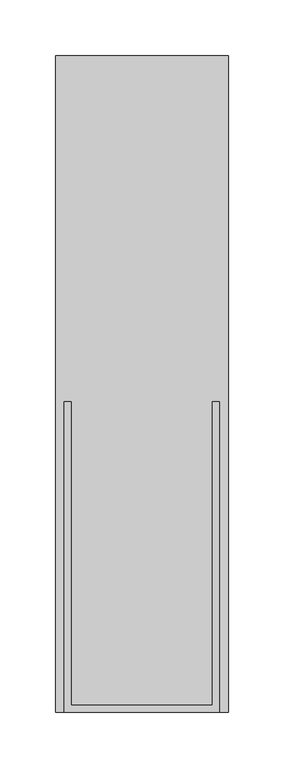
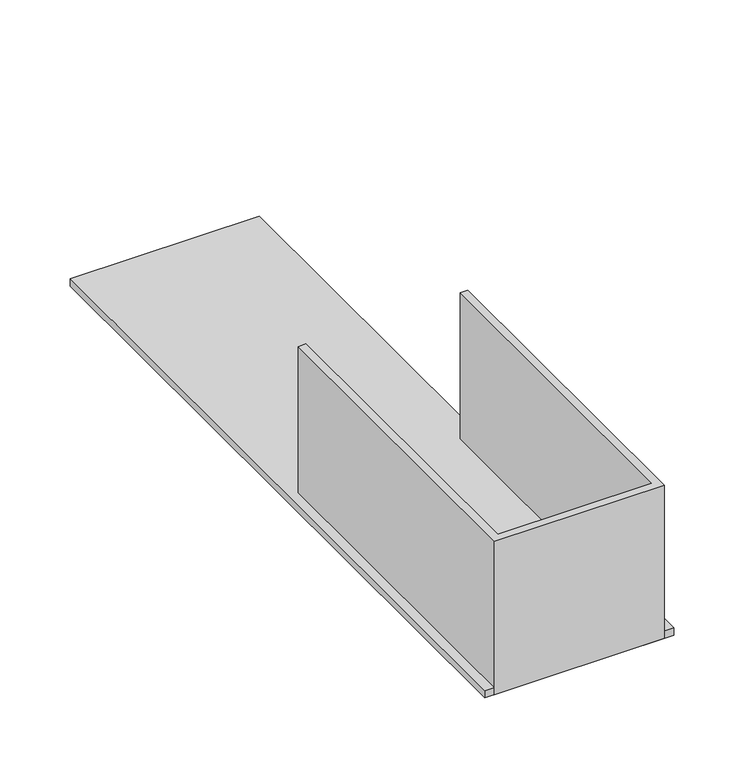
"""IFC4 building model written with IfcOpenShell, lengths in millimetres: fastener geometry, SIMPSON -THGBV - Truss Girder Hanger : SIMPSON -THGBV5.50/11 - HDG."""

from ifc_helpers import new_model, si_unit, origin, origin_with_axes, place, context, project, spatial, polyline, outline, extrude, source, transform, mapped, element, save


def fastener_118951d1(model_context):
    return source(origin(), model_context, "Body", "SweptSolid", [
        extrude(outline(polyline([(-69.85, 0.0), (-69.85, 279.4), (-63.5, 279.4), (-63.5, 6.35), (63.5, 6.35), (63.5, 279.4), (69.85, 279.4), (69.85, 0.0), (-69.85, 0.0)])), origin_with_axes(), (0.0, 0.0, 1.0), 133.35),
        extrude(outline(polyline([(77.7875, 590.55), (77.7875, 0.0), (-77.7875, 0.0), (-77.7875, 590.55), (77.7875, 590.55)])), origin_with_axes(), (0.0, 0.0, 1.0), 6.35),
    ])


if __name__ == "__main__":
    model = new_model("IFC4")
    model_context = context("Model", 3, world=origin())
    ifc_project = project(units=[si_unit("LENGTHUNIT", "METRE", prefix="MILLI")], contexts=[model_context])
    site = spatial("IfcSite", under=ifc_project)
    building = spatial("IfcBuilding", under=site)
    placement = place(None, origin())
    fastener_shape = fastener_118951d1(model_context)
    element("IfcFastener", 1, ObjectType="SIMPSON -THGBV - Truss Girder Hanger : SIMPSON -THGBV5.50/11 - HDG", at=placement, inside=building, context=model_context, shape_type="MappedRepresentation", body=[
        mapped(fastener_shape, transform((0.0, 0.0, 0.0), x_axis=(1.0, 0.0, 0.0), y_axis=(0.0, 1.0, 0.0), z_axis=(0.0, 0.0, 1.0))),
    ])
    save(model, "model.ifc")

# Revit data of these elements
# Type "SIMPSON -THGBV - Truss Girder Hanger : SIMPSON -THGBV5.50/11 - HDG"
#   URL = "http://embed.widencdn.net/pdf/plus/ssttoolbox/iecrxc4cbv/C-C-2017-p254-255.pdf"
#   W = 0' - 5 1/2"
#   H = 0' - 11"
#   Default Elevation = 4' - 0"
